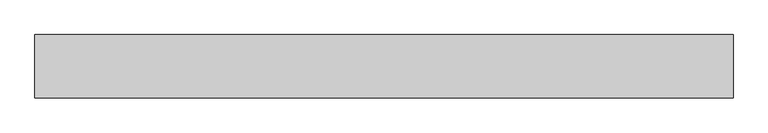
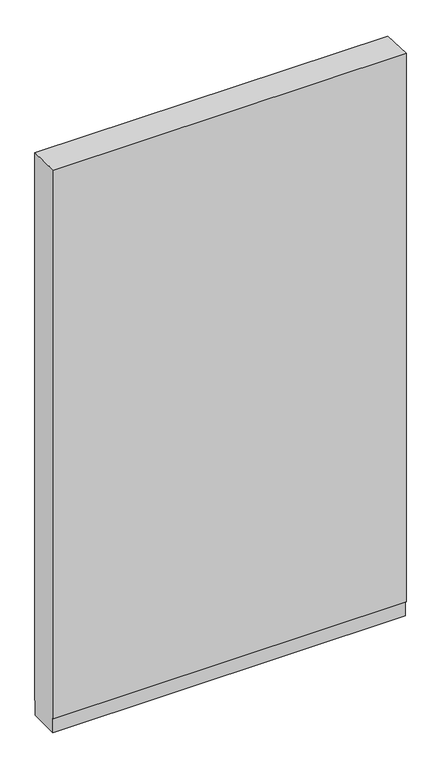
"""IFC4 building model written with IfcOpenShell, lengths in millimetres: proxy geometry, Generic Models 7:Generic Models 1:5:Generic Models 1:5 : Generic Models 7:Generic Models 1:337419:36 : Generic Models 7:Generic Models 1:5:Generic Models 1:5 : Generic Models 7:Generic Models 1:337419:311462."""

from ifc_helpers import new_model, si_unit, frame, origin, place, context, project, spatial, polyline, outline, extrude, source, transform, mapped, element, save


def generic_models_cd74a856(model_context):
    return source(origin(), model_context, "Body", "SweptSolid", [
        extrude(outline(polyline([(-530847.053884, 103.1875), (-530847.053884, 3729.5005208), (-530647.028884, 3721.1661458), (-530647.028884, 103.1875), (-530653.378884, 103.1875), (-530653.378884, 7.9375), (-530840.703884, 7.9375), (-530840.703884, 103.1875), (-530847.053884, 103.1875)])), frame((573105.3492239, 0.0, 0.0), z_axis=(1.0, 0.0, 0.0), x_axis=(0.0, 1.0, 0.0)), (0.0, 0.0, 1.0), 2205.0375),
    ])


if __name__ == "__main__":
    model = new_model("IFC4")
    model_context = context("Model", 3, world=origin())
    ifc_project = project(units=[si_unit("LENGTHUNIT", "METRE", prefix="MILLI")], contexts=[model_context])
    site = spatial("IfcSite", under=ifc_project)
    building = spatial("IfcBuilding", under=site)
    placement = place(None, origin())
    generic_models_shape = generic_models_cd74a856(model_context)
    element("IfcBuildingElementProxy", 1, Name="Generic Models 7:Generic Models 1:5:Generic Models 1:5 : Generic Models 7:Generic Models 1:337419:36 : Generic Models 7:Generic Models 1:5:Generic Models 1:5 : Generic Models 7:Generic Models 1:337419:311462", ObjectType="Generic Models 7:Generic Models 1:5:Generic Models 1:5 : Generic Models 7:Generic Models 1:337419:36 : Generic Models 7:Generic Models 1:5:Generic Models 1:5 : Generic Models 7:Generic Models 1:337419:311462", at=placement, inside=building, context=model_context, shape_type="MappedRepresentation", body=[
        mapped(generic_models_shape, transform((0.0, 0.0, 0.0), x_axis=(1.0, 0.0, 0.0), y_axis=(0.0, 1.0, 0.0), z_axis=(0.0, 0.0, 1.0))),
    ])
    save(model, "model.ifc")

# Revit data of these elements
# Type "Generic Models 7:Generic Models 1:5:Generic Models 1:5 : Generic Models 7:Generic Models 1:337419:36 : Generic Models 7:Generic Models 1:5:Generic Models 1:5 : Generic Models 7:Generic Models 1:337419:311462"
#   NameOverride = "Generic Models 7:Generic Models 1:5:Generic Models 1:5 : Generic Models 7:Generic Models 1:337419:311462"
#   ObjectTypeOverride = "Generic Models 1:5 : Generic Models 7:Generic Models 1:337419"
#   Reference = "Generic Models 1"
#   Tag = "311462"
# Element 1 (IfcBuildingElementProxy, "Generic Models 7:Generic Models 1:5:Generic Models 1:5 : Generic Models 7:Generic Models 1:337419:36 : Generic Models 7:Generic Models 1:5:Generic Models 1:5 : Generic Models 7:Generic Models 1:337419:311462")
#   Materials on its faces: "FULL CAVITY CLASS A FIBERGLASS INSULATION WITH DURABLE VAPOR BARRIER (BLACK) LINER"
# Materials
#   "FULL CAVITY CLASS A FIBERGLASS INSULATION WITH DURABLE VAPOR BARRIER (BLACK) LINER": class "Unassigned", colour RGB 158 92 175, transparency 0, Cost = 0
